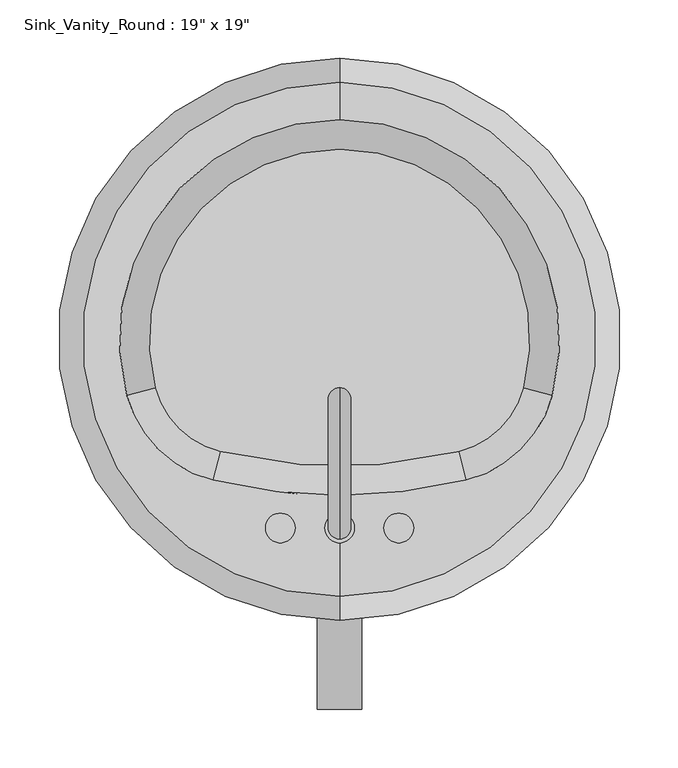
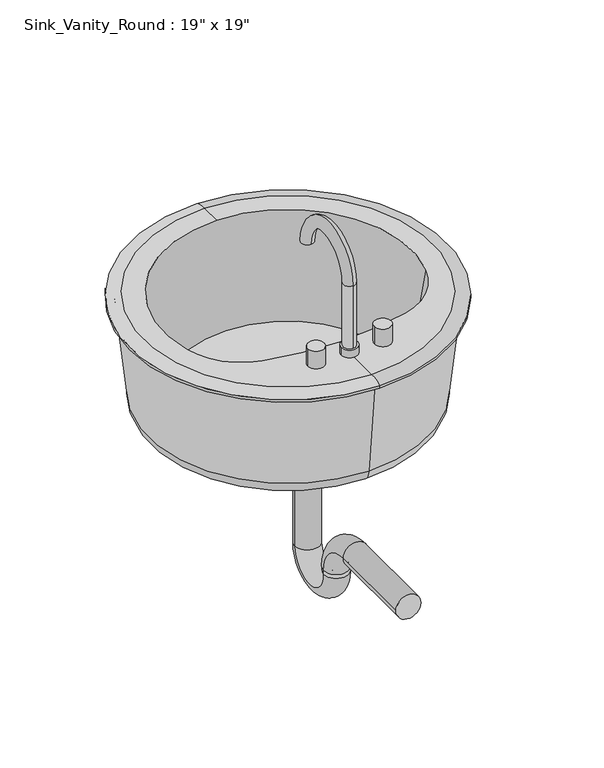
"""IFC4 building model written with IfcOpenShell, lengths in millimetres: flow terminal geometry."""

from ifc_helpers import new_model, si_unit, point, frame, frame_2d, origin, place, context, project, spatial, polyline, circle_curve, ellipse_curve, trimmed, segment, composite_curve, outline, extrude, source, transform, mapped, element, save
from ifc_brep_helpers import plane_surface, cylinder_surface, revolved_surface, advanced_brep


def flow_terminal_2c73b8fd(model_context):
    return source(origin(), model_context, "Body", "SolidModel", [
        advanced_brep(
        [(96.6517406, 135.3870093, 796.925), (96.6517406, 156.1322815, 791.36875), (96.6517406, -326.4677185, 791.36875), (96.6517406, -305.7224463, 796.925), (96.6517406, -219.2662048, 796.925), (-11.972132, -206.0284961, 796.925), (-85.8055572, -133.3356834, 796.925), (96.6517406, 103.5405705, 796.925), (279.1090383, -133.3356834, 796.925), (205.2756132, -206.0284961, 796.925), (96.6517406, 107.1264028, 615.95), (96.6517406, -85.1677185, 615.95), (96.6517406, -277.4618398, 615.95), (96.6517406, -298.0181731, 637.1342611), (96.6517406, 127.6827361, 637.1342611), (96.6517406, -314.5614685, 787.4), (96.6517406, 144.2260315, 787.4), (96.6517406, -326.4677185, 787.4), (96.6517406, 156.1322815, 787.4), (-61.2469361, -126.85231, 635.0), (-5.8718673, -181.3719195, 635.0), (199.1753484, -181.3719195, 635.0), (254.5504173, -126.85231, 635.0)],
        [
            (0, 1, circle_curve(frame((96.6517406, 139.1020246, 769.289434), z_axis=(-1.0, 0.0, 0.0), x_axis=(0.0, 1.0, 0.0)), 27.8841505)),
            (1, 2, circle_curve(frame((96.6517406, -85.1677185, 791.36875), z_axis=(0.0, 0.0, 1.0), x_axis=(0.0, -1.0, 0.0)), 241.3)),
            (2, 3, circle_curve(frame((96.6517406, -309.4374616, 769.289434), z_axis=(-1.0, 0.0, 0.0), x_axis=(0.0, -1.0, 0.0)), 27.8841505)),
            (3, 0, circle_curve(frame((96.6517406, -85.1677185, 796.925), z_axis=(0.0, 0.0, -1.0), x_axis=(0.0, -1.0, 0.0)), 220.5547278)),
            (2, 1, circle_curve(frame((96.6517406, -85.1677185, 791.36875), z_axis=(0.0, 0.0, 1.0), x_axis=(0.0, -1.0, 0.0)), 241.3)),
            (0, 3, circle_curve(frame((96.6517406, -85.1677185, 796.925), z_axis=(0.0, 0.0, -1.0), x_axis=(0.0, -1.0, 0.0)), 220.5547278)),
            (3, 4),
            (4, 5, circle_curve(frame((96.6517406, 233.0168462, 796.925), z_axis=(0.0, 0.0, -1.0), x_axis=(-0.24016790448601874, -0.9707313622495126, 0.0)), 452.283051)),
            (5, 6, circle_curve(frame((12.4289271, -107.4021897, 796.925), z_axis=(0.0, 0.0, -1.0), x_axis=(-0.9668748453196011, -0.25525092260008997, 0.0)), 101.6)),
            (6, 7, circle_curve(frame((96.6517406, -85.1677185, 796.925), z_axis=(0.0, 0.0, -1.0), x_axis=(0.9668748453195979, -0.2552509226001031, 0.0)), 188.708289)),
            (7, 0),
            (7, 8, circle_curve(frame((96.6517406, -85.1677185, 796.925), z_axis=(0.0, 0.0, -1.0), x_axis=(0.9668748453195979, -0.2552509226001031, 0.0)), 188.708289)),
            (8, 9, circle_curve(frame((180.8745541, -107.4021897, 796.925), z_axis=(0.0, 0.0, -1.0), x_axis=(0.2401679044860015, -0.970731362249517, 0.0)), 101.6)),
            (9, 4, circle_curve(frame((96.6517406, 233.0168462, 796.925), z_axis=(0.0, 0.0, -1.0), x_axis=(-0.24016790448601874, -0.9707313622495126, 0.0)), 452.283051)),
            (10, 11),
            (11, 12),
            (12, 10, circle_curve(frame((96.6517406, -85.1677185, 615.95), z_axis=(0.0, 0.0, -1.0), x_axis=(0.0, -1.0, 0.0)), 192.2941213)),
            (10, 12, circle_curve(frame((96.6517406, -85.1677185, 615.95), z_axis=(0.0, 0.0, -1.0), x_axis=(0.0, -1.0, 0.0)), 192.2941213)),
            (12, 13, circle_curve(frame((96.6517406, -277.4618398, 636.5156396), z_axis=(-1.0, 0.0, 0.0), x_axis=(0.0, -1.0, 0.0)), 20.5656396)),
            (13, 14, circle_curve(frame((96.6517406, -85.1677185, 637.1342611), z_axis=(0.0, 0.0, -1.0), x_axis=(0.0, -1.0, 0.0)), 212.8504546)),
            (14, 10, circle_curve(frame((96.6517406, 107.1264028, 636.5156396), z_axis=(-1.0, 0.0, 0.0), x_axis=(0.0, 1.0, 0.0)), 20.5656396)),
            (14, 13, circle_curve(frame((96.6517406, -85.1677185, 637.1342611), z_axis=(0.0, 0.0, -1.0), x_axis=(0.0, -1.0, 0.0)), 212.8504546)),
            (13, 15),
            (15, 16, circle_curve(frame((96.6517406, -85.1677185, 787.4), z_axis=(0.0, 0.0, -1.0), x_axis=(0.0, -1.0, 0.0)), 229.39375)),
            (16, 14),
            (16, 15, circle_curve(frame((96.6517406, -85.1677185, 787.4), z_axis=(0.0, 0.0, -1.0), x_axis=(0.0, -1.0, 0.0)), 229.39375)),
            (15, 17),
            (17, 18, circle_curve(frame((96.6517406, -85.1677185, 787.4), z_axis=(0.0, 0.0, -1.0), x_axis=(0.0, -1.0, 0.0)), 241.3)),
            (18, 16),
            (18, 17, circle_curve(frame((96.6517406, -85.1677185, 787.4), z_axis=(0.0, 0.0, -1.0), x_axis=(0.0, -1.0, 0.0)), 241.3)),
            (1, 18),
            (17, 2),
            (19, 20, circle_curve(frame((12.4289271, -107.4021897, 635.0), z_axis=(0.0, 0.0, 1.0), x_axis=(-0.9668748453196011, -0.25525092260008997, 0.0)), 76.2)),
            (20, 21, circle_curve(frame((96.6517406, 233.0168462, 635.0), z_axis=(0.0, 0.0, 1.0), x_axis=(-0.24016790448601874, -0.9707313622495126, 0.0)), 426.883051)),
            (21, 22, circle_curve(frame((180.8745541, -107.4021897, 635.0), z_axis=(0.0, 0.0, 1.0), x_axis=(0.2401679044860015, -0.970731362249517, 0.0)), 76.2)),
            (22, 19, circle_curve(frame((96.6517406, -85.1677185, 635.0), z_axis=(0.0, 0.0, 1.0), x_axis=(0.9668748453195979, -0.2552509226001031, 0.0)), 163.308289)),
            (19, 6),
            (5, 20),
            (9, 21),
            (8, 22),
        ],
        [
            revolved_surface(trimmed(ellipse_curve(frame((96.6517406, -309.4374616, 769.289434), z_axis=(-1.0, 0.0, 0.0), x_axis=(0.0, -1.0, 0.0)), 27.8841505, 27.8841505), [point((96.6517406, -326.4677185, 791.36875))], [point((96.6517406, -305.7224463, 796.925))], True, "CARTESIAN"), (96.6517406, -85.1677185, 796.925), (0.0, 0.0, 1.0)),
            plane_surface(frame((96.6517406, -85.1677185, 796.925), z_axis=(0.0, 0.0, 1.0), x_axis=(0.0, -1.0, 0.0))),
            plane_surface(frame((96.6517406, -85.1677185, 615.95), z_axis=(0.0, 0.0, -1.0), x_axis=(0.0, -1.0, 0.0))),
            revolved_surface(trimmed(ellipse_curve(frame((96.6517406, -277.4618398, 636.5156396), z_axis=(-1.0, 0.0, 0.0), x_axis=(0.0, -1.0, 0.0)), 20.5656396, 20.5656396), [point((96.6517406, -277.4618398, 615.95))], [point((96.6517406, -298.0181731, 637.1342611))], True, "CARTESIAN"), (96.6517406, -85.1677185, 796.925), (0.0, 0.0, 1.0)),
            revolved_surface(polyline([(96.6517406, -298.0181731, 637.1342611), (96.6517406, -314.5614685, 787.4)]), (96.6517406, -85.1677185, 796.925), (0.0, 0.0, 1.0)),
            plane_surface(frame((96.6517406, -85.1677185, 787.4), z_axis=(0.0, 0.0, -1.0), x_axis=(0.0, -1.0, 0.0))),
            cylinder_surface(frame((96.6517406, -85.1677185, 796.925), z_axis=(0.0, 0.0, 1.0), x_axis=(0.0, -1.0, 0.0)), 241.3),
            plane_surface(frame((96.6517406, -154.1121147, 635.0), z_axis=(0.0, 0.0, 1.0), x_axis=(-0.2552509226000978, 0.9668748453195992, 0.0))),
            revolved_surface(polyline([(-85.8055572, -133.3356834, 796.925), (-61.246936125000005, -126.852309975, 635.0)]), (12.4289271, -107.4021897, 149.225), (0.0, 0.0, 1.0)),
            revolved_surface(polyline([(-11.972132000000002, -206.0284961, 796.9250000000002), (-5.871867225621074, -181.3719194941331, 635.0)]), (96.6517406, 233.0168462, -2086.3794501), (0.0, 0.0, 1.0)),
            revolved_surface(polyline([(205.2756132, -206.0284961, 796.925), (199.175348425, -181.3719195, 635.0)]), (180.8745541, -107.4021897, 149.225), (0.0, 0.0, 1.0)),
            revolved_surface(polyline([(279.1090383, -133.3356834, 796.925), (254.55041724055098, -126.85230996360858, 635.0)]), (96.6517406, -85.1677185, -406.0903427), (0.0, 0.0, 1.0)),
        ],
        [
            (0, [[1, 2, 3, 4]]),
            (0, [[5, -1, 6, -3]]),
            (1, [[7, 8, 9, 10, 11, -4]]),
            (1, [[-11, 12, 13, 14, -7, -6]]),
            (2, [[15, 16, 17]]),
            (2, [[-15, 18, -16]]),
            (3, [[19, 20, 21, -17]]),
            (3, [[-21, 22, -19, -18]]),
            (4, [[23, 24, 25, -20]]),
            (4, [[-25, 26, -23, -22]]),
            (5, [[27, 28, 29, -24]]),
            (5, [[-29, 30, -27, -26]]),
            (6, [[31, -28, 32, -2]]),
            (6, [[-32, -30, -31, -5]]),
            (7, [[33, 34, 35, 36]]),
            (8, [[37, -9, 38, -33]]),
            (9, [[-38, -8, -14, 39, -34]]),
            (10, [[-39, -13, 40, -35]]),
            (11, [[-40, -12, -10, -37, -36]]),
        ],
    ),
        advanced_brep(
        [(83.9517406, -247.0927185, 796.925), (109.3517406, -247.0927185, 796.925), (96.6517406, -237.5677185, 909.6375), (96.6517406, -237.5677185, 809.625), (96.6517406, -256.6177185, 809.625), (96.6517406, -256.6177185, 909.6375), (96.6517406, -145.7775038, 909.6375), (96.6517406, -126.7275038, 909.6375), (83.9517406, -247.0927185, 809.625), (109.3517406, -247.0927185, 809.625)],
        [
            (0, 1, circle_curve(frame((96.6517406, -247.0927185, 796.925), z_axis=(0.0, 0.0, -1.0), x_axis=(1.0, 0.0, 0.0)), 12.7)),
            (1, 0, circle_curve(frame((96.6517406, -247.0927185, 796.925), z_axis=(0.0, 0.0, -1.0), x_axis=(1.0, 0.0, 0.0)), 12.7)),
            (2, 3),
            (3, 4, circle_curve(frame((96.6517406, -247.0927185, 809.625), z_axis=(0.0, 0.0, 1.0), x_axis=(0.0, -1.0, 0.0)), 9.525)),
            (4, 5),
            (5, 2, circle_curve(frame((96.6517406, -247.0927185, 909.6375), z_axis=(0.0, 0.0, -1.0), x_axis=(0.0, -1.0, 0.0)), 9.525)),
            (4, 3, circle_curve(frame((96.6517406, -247.0927185, 809.625), z_axis=(0.0, 0.0, 1.0), x_axis=(0.0, -1.0, 0.0)), 9.525)),
            (2, 5, circle_curve(frame((96.6517406, -247.0927185, 909.6375), z_axis=(0.0, 0.0, -1.0), x_axis=(0.0, -1.0, 0.0)), 9.525)),
            (6, 7, circle_curve(frame((96.6517406, -136.2525038, 909.6375), z_axis=(0.0, 0.0, -1.0), x_axis=(0.0, 1.0, 0.0)), 9.525)),
            (7, 6, circle_curve(frame((96.6517406, -136.2525038, 909.6375), z_axis=(0.0, 0.0, -1.0), x_axis=(0.0, 1.0, 0.0)), 9.525)),
            (5, 7, circle_curve(frame((96.6517406, -191.6726112, 909.6375), z_axis=(-1.0, 0.0, 0.0), x_axis=(0.0, -1.0, 0.0)), 64.9451073)),
            (6, 2, circle_curve(frame((96.6517406, -191.6726112, 909.6375), z_axis=(1.0, 0.0, 0.0), x_axis=(0.0, -1.0, 0.0)), 45.8951073)),
            (8, 9, circle_curve(frame((96.6517406, -247.0927185, 809.625), z_axis=(0.0, 0.0, 1.0), x_axis=(1.0, 0.0, 0.0)), 12.7)),
            (9, 8, circle_curve(frame((96.6517406, -247.0927185, 809.625), z_axis=(0.0, 0.0, 1.0), x_axis=(1.0, 0.0, 0.0)), 12.7)),
            (9, 1),
            (0, 8),
        ],
        [
            plane_surface(frame((96.6517406, -237.5677185, 796.925), z_axis=(0.0, 0.0, -1.0), x_axis=(1.0, 0.0, 0.0))),
            cylinder_surface(frame((96.6517406, -247.0927185, 796.925), z_axis=(0.0, 0.0, -1.0), x_axis=(0.0, -1.0, 0.0)), 9.525),
            plane_surface(frame((96.6517406, -191.6726112, 909.6375), z_axis=(0.0, 0.0, -1.0), x_axis=(0.0, 1.0, 0.0))),
            revolved_surface(trimmed(ellipse_curve(frame((96.6517406, -247.0927185, 909.6375), z_axis=(0.0, 0.0, 1.0), x_axis=(0.0, -1.0, 0.0)), 9.525, 9.525), [point((96.6517406, -237.5677185, 909.6375))], [point((96.6517406, -256.6177185, 909.6375))], True, "CARTESIAN"), (96.6517406, -191.6726112, 909.6375), (1.0, 0.0, 0.0)),
            revolved_surface(trimmed(ellipse_curve(frame((96.6517406, -247.0927185, 909.6375), z_axis=(0.0, 0.0, 1.0), x_axis=(0.0, -1.0, 0.0)), 9.525, 9.525), [point((96.6517406, -256.6177185, 909.6375))], [point((96.6517406, -237.5677185, 909.6375))], True, "CARTESIAN"), (96.6517406, -191.6726112, 909.6375), (1.0, 0.0, 0.0)),
            plane_surface(frame((109.3517406, -247.0927185, 809.625), z_axis=(0.0, 0.0, 1.0), x_axis=(0.0, -1.0, 0.0))),
            cylinder_surface(frame((96.6517406, -247.0927185, 796.925), z_axis=(0.0, 0.0, 1.0), x_axis=(1.0, 0.0, 0.0)), 12.7),
        ],
        [
            (0, [[1, 2]]),
            (1, [[3, 4, 5, 6]]),
            (1, [[-5, 7, -3, 8]]),
            (2, [[9, 10]]),
            (3, [[11, -9, 12, -6]]),
            (4, [[-12, -10, -11, -8]]),
            (5, [[13, 14], [-7, -4]]),
            (6, [[15, -1, 16, -14]]),
            (6, [[-16, -2, -15, -13]]),
        ],
    ),
        extrude(outline(composite_curve([segment(trimmed(circle_curve(frame_2d((45.8517406, -247.0927185)), 12.7), [point((33.1517406, -247.0927185))], [point((58.5517406, -247.0927185))], False, "CARTESIAN"), True, "CONTINUOUS"), segment(trimmed(circle_curve(frame_2d((45.8517406, -247.0927185)), 12.7), [point((58.5517406, -247.0927185))], [point((33.1517406, -247.0927185))], False, "CARTESIAN"), True, "CONTINUOUS")], self_intersect=False)), frame((0.0, 0.0, 796.925), z_axis=(0.0, 0.0, 1.0), x_axis=(1.0, 0.0, 0.0)), (0.0, 0.0, 1.0), 28.575),
        extrude(outline(composite_curve([segment(trimmed(circle_curve(frame_2d((147.4517406, -247.0927185)), 12.7), [point((134.7517406, -247.0927185))], [point((160.1517406, -247.0927185))], False, "CARTESIAN"), True, "CONTINUOUS"), segment(trimmed(circle_curve(frame_2d((147.4517406, -247.0927185)), 12.7), [point((160.1517406, -247.0927185))], [point((134.7517406, -247.0927185))], False, "CARTESIAN"), True, "CONTINUOUS")], self_intersect=False)), frame((0.0, 0.0, 796.925), z_axis=(0.0, 0.0, 1.0), x_axis=(1.0, 0.0, 0.0)), (0.0, 0.0, 1.0), 28.575),
        advanced_brep(
        [(77.6017406, -135.9677185, 615.95), (115.7017406, -135.9677185, 615.95), (115.7017406, -135.9677185, 425.45), (77.6017406, -135.9677185, 425.45), (115.7017406, -212.1677185, 425.45), (77.6017406, -212.1677185, 425.45), (115.7017406, -212.1677185, 431.8), (77.6017406, -212.1677185, 431.8), (115.7017406, -262.9677185, 482.6), (77.6017406, -262.9677185, 482.6), (77.6017406, -402.6677185, 482.6), (115.7017406, -402.6677185, 482.6)],
        [
            (0, 1, circle_curve(frame((96.6517406, -135.9677185, 615.95), z_axis=(0.0, 0.0, 1.0), x_axis=(1.0, 0.0, 0.0)), 19.05)),
            (1, 0, circle_curve(frame((96.6517406, -135.9677185, 615.95), z_axis=(0.0, 0.0, 1.0), x_axis=(1.0, 0.0, 0.0)), 19.05)),
            (1, 2),
            (2, 3, circle_curve(frame((96.6517406, -135.9677185, 425.45), z_axis=(0.0, 0.0, 1.0), x_axis=(1.0, 0.0, 0.0)), 19.05)),
            (3, 0),
            (3, 2, circle_curve(frame((96.6517406, -135.9677185, 425.45), z_axis=(0.0, 0.0, 1.0), x_axis=(1.0, 0.0, 0.0)), 19.05)),
            (4, 5, circle_curve(frame((96.6517406, -212.1677185, 425.45), z_axis=(0.0, 0.0, -1.0), x_axis=(1.0, 0.0, 0.0)), 19.05)),
            (5, 3, circle_curve(frame((77.6017406, -174.0677185, 425.45), z_axis=(1.0, 0.0, 0.0), x_axis=(0.0, 1.0, 0.0)), 38.1)),
            (2, 4, circle_curve(frame((115.7017406, -174.0677185, 425.45), z_axis=(-1.0, 0.0, 0.0), x_axis=(0.0, 1.0, 0.0)), 38.1)),
            (5, 4, circle_curve(frame((96.6517406, -212.1677185, 425.45), z_axis=(0.0, 0.0, -1.0), x_axis=(1.0, 0.0, 0.0)), 19.05)),
            (4, 6),
            (6, 7, circle_curve(frame((96.6517406, -212.1677185, 431.8), z_axis=(0.0, 0.0, -1.0), x_axis=(1.0, 0.0, 0.0)), 19.05)),
            (7, 5),
            (7, 6, circle_curve(frame((96.6517406, -212.1677185, 431.8), z_axis=(0.0, 0.0, -1.0), x_axis=(1.0, 0.0, 0.0)), 19.05)),
            (8, 9, circle_curve(frame((96.6517406, -262.9677185, 482.6), z_axis=(0.0, 1.0, 0.0), x_axis=(1.0, 0.0, 0.0)), 19.05)),
            (9, 7, circle_curve(frame((77.6017406, -262.9677185, 431.8), z_axis=(-1.0, 0.0, 0.0), x_axis=(0.0, 1.0, 0.0)), 50.8)),
            (6, 8, circle_curve(frame((115.7017406, -262.9677185, 431.8), z_axis=(1.0, 0.0, 0.0), x_axis=(0.0, 1.0, 0.0)), 50.8)),
            (9, 8, circle_curve(frame((96.6517406, -262.9677185, 482.6), z_axis=(0.0, 1.0, 0.0), x_axis=(1.0, 0.0, 0.0)), 19.05)),
            (10, 11, circle_curve(frame((96.6517406, -402.6677185, 482.6), z_axis=(0.0, -1.0, 0.0), x_axis=(1.0, 0.0, 0.0)), 19.05)),
            (11, 10, circle_curve(frame((96.6517406, -402.6677185, 482.6), z_axis=(0.0, -1.0, 0.0), x_axis=(1.0, 0.0, 0.0)), 19.05)),
            (8, 11),
            (10, 9),
        ],
        [
            plane_surface(frame((96.6517406, -135.9677185, 615.95), z_axis=(0.0, 0.0, 1.0), x_axis=(1.0, 0.0, 0.0))),
            cylinder_surface(frame((96.6517406, -135.9677185, 615.95), z_axis=(0.0, 0.0, 1.0), x_axis=(1.0, 0.0, 0.0)), 19.05),
            revolved_surface(trimmed(ellipse_curve(frame((96.6517406, -135.9677185, 425.45), z_axis=(0.0, 0.0, -1.0), x_axis=(1.0, 0.0, 0.0)), 19.05, 19.05), [point((77.6017406, -135.9677185, 425.45))], [point((115.7017406, -135.9677185, 425.45))], True, "CARTESIAN"), (96.6517406, -174.0677185, 425.45), (1.0, 0.0, 0.0)),
            revolved_surface(trimmed(ellipse_curve(frame((96.6517406, -135.9677185, 425.45), z_axis=(0.0, 0.0, -1.0), x_axis=(1.0, 0.0, 0.0)), 19.05, 19.05), [point((115.7017406, -135.9677185, 425.45))], [point((77.6017406, -135.9677185, 425.45))], True, "CARTESIAN"), (96.6517406, -174.0677185, 425.45), (1.0, 0.0, 0.0)),
            cylinder_surface(frame((96.6517406, -212.1677185, 425.45), z_axis=(0.0, 0.0, -1.0), x_axis=(1.0, 0.0, 0.0)), 19.05),
            revolved_surface(trimmed(ellipse_curve(frame((96.6517406, -212.1677185, 431.8), z_axis=(0.0, 0.0, 1.0), x_axis=(1.0, 0.0, 0.0)), 19.05, 19.05), [point((77.6017406, -212.1677185, 431.8))], [point((115.7017406, -212.1677185, 431.8))], True, "CARTESIAN"), (96.6517406, -262.9677185, 431.8), (-1.0, 0.0, 0.0)),
            revolved_surface(trimmed(ellipse_curve(frame((96.6517406, -212.1677185, 431.8), z_axis=(0.0, 0.0, 1.0), x_axis=(1.0, 0.0, 0.0)), 19.05, 19.05), [point((115.7017406, -212.1677185, 431.8))], [point((77.6017406, -212.1677185, 431.8))], True, "CARTESIAN"), (96.6517406, -262.9677185, 431.8), (-1.0, 0.0, 0.0)),
            plane_surface(frame((96.6517406, -402.6677185, 482.6), z_axis=(0.0, -1.0, 0.0), x_axis=(1.0, 0.0, 0.0))),
            cylinder_surface(frame((96.6517406, -262.9677185, 482.6), z_axis=(0.0, 1.0, 0.0), x_axis=(1.0, 0.0, 0.0)), 19.05),
        ],
        [
            (0, [[1, 2]]),
            (1, [[3, 4, 5, -2]]),
            (1, [[-5, 6, -3, -1]]),
            (2, [[7, 8, -4, 9]]),
            (3, [[10, -9, -6, -8]]),
            (4, [[11, 12, 13, -7]]),
            (4, [[-13, 14, -11, -10]]),
            (5, [[15, 16, -12, 17]]),
            (6, [[18, -17, -14, -16]]),
            (7, [[19, 20]]),
            (8, [[21, -19, 22, -15]]),
            (8, [[-22, -20, -21, -18]]),
        ],
    ),
    ])


if __name__ == "__main__":
    model = new_model("IFC4")
    model_context = context("Model", 3, world=origin())
    ifc_project = project(units=[si_unit("LENGTHUNIT", "METRE", prefix="MILLI")], contexts=[model_context])
    site = spatial("IfcSite", under=ifc_project)
    building = spatial("IfcBuilding", under=site)
    placement = place(None, origin())
    flow_terminal_shape = flow_terminal_2c73b8fd(model_context)
    element("IfcFlowTerminal", 1, ObjectType="Sink_Vanity_Round : 19\" x 19\"", at=placement, inside=building, context=model_context, shape_type="MappedRepresentation", body=[
        mapped(flow_terminal_shape, transform((0.0, 0.0, 0.0), x_axis=(1.0, 0.0, 0.0), y_axis=(0.0, 1.0, 0.0), z_axis=(0.0, 0.0, 1.0))),
    ])
    save(model, "model.ifc")

# Revit data of these elements
# Type "Sink_Vanity_Round : 19\" x 19\""
#   Assembly Code = "D2010400"
#   Top Of Counter = 2' - 7"
#   Basin Material = Fixtures - Porcelain - Linen
#   Faucet Material = Fixtures - Metal - Chrome
# Element 1 (IfcFlowTerminal, "Sink_Vanity_Round : 19\" x 19\"")
#   Materials on its faces: "Fixtures - Metal - Chrome", "Fixtures - Porcelain - Linen"
# Materials
#   "Fixtures - Porcelain - Linen": class "Unassigned", colour RGB 249 239 230, transparency 0, Keynote = "15410", Description = "Porcelain Sinks and Water Closets"
#   "Fixtures - Metal - Chrome": class "Unassigned", colour RGB 247 247 247, transparency 0, Description = "Chrome finished Plumbing Fixtures"
